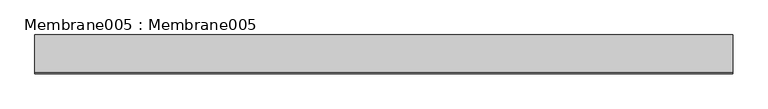
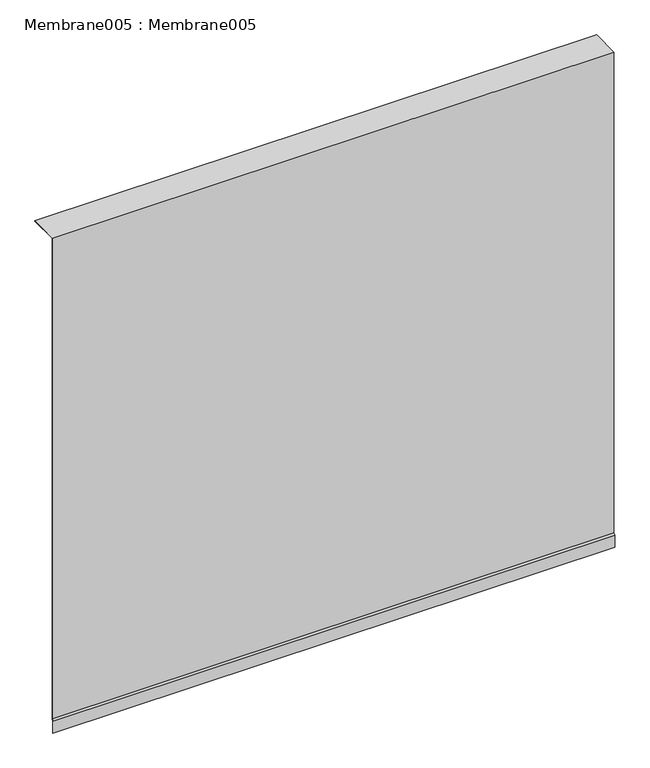
"""IFC4 building model written with IfcOpenShell, lengths in millimetres: proxy geometry, Membrane005 : Membrane005."""

from ifc_helpers import new_model, si_unit, frame, origin, place, context, project, spatial, polyline, outline, extrude, source, transform, mapped, element, save


def membrane005_membrane005_daeb98a2(model_context):
    return source(origin(), model_context, "Body", "SweptSolid", [
        extrude(outline(polyline([(-4662.0876539, 36597.8828125), (-4662.0876539, 36553.203125), (-4663.5876539, 36553.203125), (-4663.5876539, 36598.2944693), (-4659.4279428, 36605.3022818), (-4659.4279428, 38413.7101562), (-4552.1284743, 38413.7101562), (-4552.1284743, 38412.2101562), (-4657.9279428, 38412.2101562), (-4657.9279428, 36604.890625), (-4662.0876539, 36597.8828125)])), frame((12383.0178845, 0.0, 0.0), z_axis=(1.0, 0.0, 0.0), x_axis=(0.0, 1.0, 0.0)), (0.0, 0.0, 1.0), 2000.0),
    ])


if __name__ == "__main__":
    model = new_model("IFC4")
    model_context = context("Model", 3, world=origin())
    ifc_project = project(units=[si_unit("LENGTHUNIT", "METRE", prefix="MILLI")], contexts=[model_context])
    site = spatial("IfcSite", under=ifc_project)
    building = spatial("IfcBuilding", under=site)
    placement = place(None, origin())
    membrane005_membrane005_shape = membrane005_membrane005_daeb98a2(model_context)
    element("IfcBuildingElementProxy", 1, Name="Membrane005 : Membrane005", ObjectType="Membrane005 : Membrane005", at=placement, inside=building, context=model_context, shape_type="MappedRepresentation", body=[
        mapped(membrane005_membrane005_shape, transform((0.0, 0.0, 0.0), x_axis=(1.0, 0.0, 0.0), y_axis=(0.0, 1.0, 0.0), z_axis=(0.0, 0.0, 1.0))),
    ])
    save(model, "model.ifc")

# Revit data of these elements
# Type "Membrane005 : Membrane005"
#   NameOverride = "Membrane005"
# Element 1 (IfcBuildingElementProxy, "Membrane005 : Membrane005")
#   Materials on its faces: "(2) LAYERS OF ICE & WATER SHIELD (BITUTHANE) UNDER STUCCO"
# Materials
#   "(2) LAYERS OF ICE & WATER SHIELD (BITUTHANE) UNDER STUCCO": class "Unassigned", colour RGB 186 255 159, transparency 0, Cost = 0
